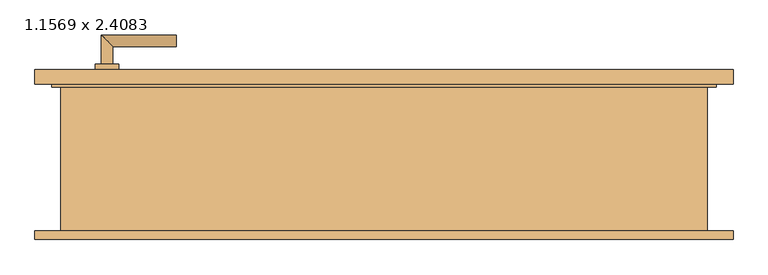
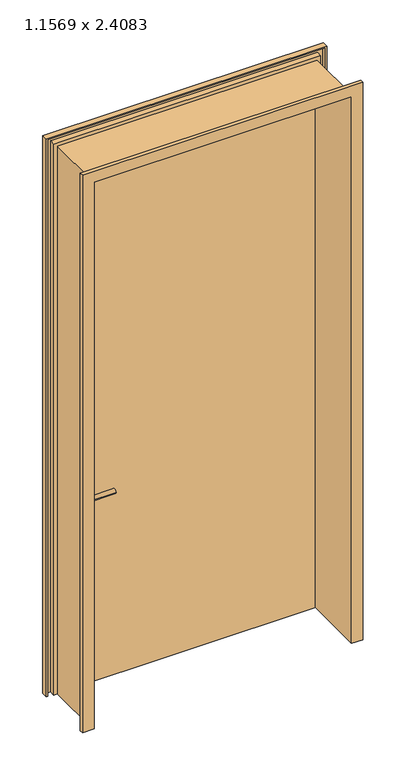
"""IFC4 building model written with IfcOpenShell, lengths in millimetres: door geometry, Drehflügel 1-flg - Stahlzarge : 1.1569 x 2.4083."""

from ifc_helpers import new_model, si_unit, point, frame, frame_2d, origin, place, context, project, spatial, polyline, circle_curve, ellipse_curve, trimmed, segment, composite_curve, outline, extrude, faceted_brep, source, transform, mapped, element, save
from ifc_brep_helpers import plane_surface, cylinder_surface, advanced_brep


def door_1_1569_x_2_4083_937cce7c(model_context):
    return source(origin(), model_context, "Body", "SolidModel", [
        advanced_brep(
        [(-488.45, 116.4346141, 1000.0), (-468.45, 116.4346141, 1000.0), (-488.45, 46.4346141, 1000.0), (-468.45, 66.4346141, 1000.0), (-358.45, 46.4346141, 1000.0), (-358.45, 66.4346141, 1000.0)],
        [
            (0, 1, circle_curve(frame((-478.45, 116.4346141, 1000.0), z_axis=(0.0, 1.0, 0.0), x_axis=(1.0, 0.0, 0.0)), 10.0)),
            (1, 0, circle_curve(frame((-478.45, 116.4346141, 1000.0), z_axis=(0.0, 1.0, 0.0), x_axis=(1.0, 0.0, 0.0)), 10.0)),
            (0, 2),
            (2, 3, ellipse_curve(frame((-478.45, 56.4346141, 1000.0), z_axis=(-0.7071067811865385, 0.7071067811865565, 0.0), x_axis=(0.7071067811865563, 0.7071067811865386, 0.0)), 14.1421356, 10.0)),
            (3, 1),
            (3, 2, ellipse_curve(frame((-478.45, 56.4346141, 1000.0), z_axis=(-0.7071067811865385, 0.7071067811865565, 0.0), x_axis=(0.7071067811865563, 0.7071067811865386, 0.0)), 14.1421356, 10.0)),
            (4, 5, circle_curve(frame((-358.45, 56.4346141, 1000.0), z_axis=(1.0, 0.0, 0.0), x_axis=(0.0, 1.0, 0.0)), 10.0)),
            (5, 4, circle_curve(frame((-358.45, 56.4346141, 1000.0), z_axis=(1.0, 0.0, 0.0), x_axis=(0.0, 1.0, 0.0)), 10.0)),
            (2, 4),
            (5, 3),
        ],
        [
            plane_surface(frame((-478.45, 116.4346141, -287.7526403), z_axis=(0.0, 1.0, 0.0), x_axis=(0.0, 0.0, 1.0))),
            cylinder_surface(frame((-478.45, 116.4346141, 1000.0), z_axis=(0.0, 1.0, 0.0), x_axis=(1.0, 0.0, 0.0)), 10.0),
            plane_surface(frame((-358.45, 56.4346141, -287.7526403), z_axis=(1.0, 0.0, 0.0), x_axis=(0.0, 0.0, 1.0))),
            cylinder_surface(frame((-478.45, 56.4346141, 1000.0), z_axis=(-1.0, 0.0, 0.0), x_axis=(0.0, 1.0, 0.0)), 10.0),
        ],
        [
            (0, [[1, 2]]),
            (1, [[-1, 3, 4, 5]]),
            (1, [[-2, -5, 6, -3]]),
            (2, [[7, 8]]),
            (3, [[-4, 9, -8, 10]]),
            (3, [[-6, -10, -7, -9]]),
        ],
    ),
        advanced_brep(
        [(-468.45, 176.4346141, 1000.0), (-488.45, 176.4346141, 1000.0), (-468.45, 206.4346141, 1000.0), (-488.45, 226.4346141, 1000.0), (-358.45, 206.4346141, 1000.0), (-358.45, 226.4346141, 1000.0)],
        [
            (0, 1, circle_curve(frame((-478.45, 176.4346141, 1000.0), z_axis=(0.0, -1.0, 0.0), x_axis=(-1.0, 0.0, 0.0)), 10.0)),
            (1, 0, circle_curve(frame((-478.45, 176.4346141, 1000.0), z_axis=(0.0, -1.0, 0.0), x_axis=(-1.0, 0.0, 0.0)), 10.0)),
            (0, 2),
            (2, 3, ellipse_curve(frame((-478.45, 216.4346141, 1000.0), z_axis=(-0.7071067811865475, -0.7071067811865475, 0.0), x_axis=(0.7071067811865474, -0.7071067811865476, 0.0)), 14.1421356, 10.0)),
            (3, 1),
            (3, 2, ellipse_curve(frame((-478.45, 216.4346141, 1000.0), z_axis=(-0.7071067811865475, -0.7071067811865475, 0.0), x_axis=(0.7071067811865474, -0.7071067811865476, 0.0)), 14.1421356, 10.0)),
            (4, 5, circle_curve(frame((-358.45, 216.4346141, 1000.0), z_axis=(1.0, 0.0, 0.0), x_axis=(0.0, 1.0, 0.0)), 10.0)),
            (5, 4, circle_curve(frame((-358.45, 216.4346141, 1000.0), z_axis=(1.0, 0.0, 0.0), x_axis=(0.0, 1.0, 0.0)), 10.0)),
            (2, 4),
            (5, 3),
        ],
        [
            plane_surface(frame((-478.45, 176.4346141, -287.7526403), z_axis=(0.0, -1.0, 0.0), x_axis=(0.0, 0.0, 1.0))),
            cylinder_surface(frame((-478.45, 176.4346141, 1000.0), z_axis=(0.0, -1.0, 0.0), x_axis=(-1.0, 0.0, 0.0)), 10.0),
            plane_surface(frame((-358.45, 216.4346141, -287.7526403), z_axis=(1.0, 0.0, 0.0), x_axis=(0.0, 0.0, 1.0))),
            cylinder_surface(frame((-478.45, 216.4346141, 1000.0), z_axis=(-1.0, 0.0, 0.0), x_axis=(0.0, 1.0, 0.0)), 10.0),
        ],
        [
            (0, [[1, 2]]),
            (1, [[-1, 3, 4, 5]]),
            (1, [[-2, -5, 6, -3]]),
            (2, [[7, 8]]),
            (3, [[-4, 9, -8, 10]]),
            (3, [[-6, -10, -7, -9]]),
        ],
    ),
        extrude(outline(composite_curve([segment(trimmed(circle_curve(frame_2d((1000.0, -478.45)), 20.0), [point((1000.0, -498.45))], [point((1000.0, -458.45))], False, "CARTESIAN"), True, "CONTINUOUS"), segment(trimmed(circle_curve(frame_2d((1000.0, -478.45)), 20.0), [point((1000.0, -458.45))], [point((1000.0, -498.45))], False, "CARTESIAN"), True, "CONTINUOUS")], self_intersect=False)), frame((0.0, 106.4346141, 0.0), z_axis=(0.0, 1.0, 0.0), x_axis=(0.0, 0.0, 1.0)), (0.0, 0.0, 1.0), 10.0),
        extrude(outline(composite_curve([segment(trimmed(circle_curve(frame_2d((1000.0, -478.45)), 20.0), [point((1000.0, -498.45))], [point((1000.0, -458.45))], False, "CARTESIAN"), True, "CONTINUOUS"), segment(trimmed(circle_curve(frame_2d((1000.0, -478.45)), 20.0), [point((1000.0, -458.45))], [point((1000.0, -498.45))], False, "CARTESIAN"), True, "CONTINUOUS")], self_intersect=False)), frame((0.0, 166.4346141, 0.0), z_axis=(0.0, 1.0, 0.0), x_axis=(0.0, 0.0, 1.0)), (0.0, 0.0, 1.0), 10.0),
        extrude(outline(polyline([(568.45, 141.4346141), (-568.45, 141.4346141), (-568.45, 166.4346141), (568.45, 166.4346141), (568.45, 141.4346141)])), frame((0.0, 0.0, 100.0), z_axis=(0.0, 0.0, 1.0), x_axis=(1.0, 0.0, 0.0)), (0.0, 0.0, 1.0), 2498.3),
        faceted_brep([(602.9103207, -127.5653859, 100.0), (553.45, -127.5653859, 100.0), (553.45, 141.4346141, 100.0), (568.45, 141.4346141, 100.0), (568.45, 166.4346141, 100.0), (602.9103207, 166.4346141, 100.0), (602.9103207, 141.4346141, 100.0), (597.9103207, 141.4346141, 100.0), (597.9103207, 161.4346141, 100.0), (573.45, 161.4346141, 100.0), (573.45, 136.4346141, 100.0), (558.45, 136.4346141, 100.0), (558.45, -122.5653859, 100.0), (597.9103207, -122.5653859, 100.0), (597.9103207, -112.5653859, 100.0), (602.9103207, -112.5653859, 100.0), (602.9103207, -127.5653859, 2632.7603207), (-602.9103207, -127.5653859, 2632.7603207), (-602.9103207, -127.5653859, 100.0), (-553.45, -127.5653859, 100.0), (-553.45, -127.5653859, 2583.3), (553.45, -127.5653859, 2583.3), (553.45, 141.4346141, 2583.3), (-553.45, 141.4346141, 2583.3), (-553.45, 141.4346141, 100.0), (-568.45, 141.4346141, 100.0), (-568.45, 141.4346141, 2598.3), (568.45, 141.4346141, 2598.3), (568.45, 166.4346141, 2598.3), (-568.45, 166.4346141, 2598.3), (-568.45, 166.4346141, 100.0), (-602.9103207, 166.4346141, 100.0), (-602.9103207, 166.4346141, 2632.7603207), (602.9103207, 166.4346141, 2632.7603207), (602.9103207, 141.4346141, 2632.7603207), (-602.9103207, 141.4346141, 2632.7603207), (-602.9103207, 141.4346141, 100.0), (-597.9103207, 141.4346141, 100.0), (-597.9103207, 141.4346141, 2627.7603207), (597.9103207, 141.4346141, 2627.7603207), (597.9103207, 161.4346141, 2627.7603207), (-597.9103207, 161.4346141, 2627.7603207), (-597.9103207, 161.4346141, 100.0), (-573.45, 161.4346141, 100.0), (-573.45, 161.4346141, 2603.3), (573.45, 161.4346141, 2603.3), (573.45, 136.4346141, 2603.3), (-573.45, 136.4346141, 2603.3), (-573.45, 136.4346141, 100.0), (-558.45, 136.4346141, 100.0), (-558.45, 136.4346141, 2588.3), (558.45, 136.4346141, 2588.3), (558.45, -122.5653859, 2588.3), (-558.45, -122.5653859, 2588.3), (-558.45, -122.5653859, 100.0), (-597.9103207, -122.5653859, 100.0), (-597.9103207, -122.5653859, 2627.7603207), (597.9103207, -122.5653859, 2627.7603207), (597.9103207, -112.5653859, 2627.7603207), (-597.9103207, -112.5653859, 2627.7603207), (-597.9103207, -112.5653859, 100.0), (-602.9103207, -112.5653859, 100.0), (-602.9103207, -112.5653859, 2632.7603207), (602.9103207, -112.5653859, 2632.7603207)], [[[0, 1, 2, 3, 4, 5, 6, 7, 8, 9, 10, 11, 12, 13, 14, 15]], [[1, 0, 16, 17, 18, 19, 20, 21]], [[2, 1, 21, 22]], [[3, 2, 22, 23, 24, 25, 26, 27]], [[4, 3, 27, 28]], [[5, 4, 28, 29, 30, 31, 32, 33]], [[6, 5, 33, 34]], [[7, 6, 34, 35, 36, 37, 38, 39]], [[8, 7, 39, 40]], [[9, 8, 40, 41, 42, 43, 44, 45]], [[10, 9, 45, 46]], [[11, 10, 46, 47, 48, 49, 50, 51]], [[12, 11, 51, 52]], [[13, 12, 52, 53, 54, 55, 56, 57]], [[14, 13, 57, 58]], [[15, 14, 58, 59, 60, 61, 62, 63]], [[0, 15, 63, 16]], [[17, 62, 61, 18]], [[18, 61, 60, 55, 54, 49, 48, 43, 42, 37, 36, 31, 30, 25, 24, 19]], [[23, 20, 19, 24]], [[29, 26, 25, 30]], [[35, 32, 31, 36]], [[41, 38, 37, 42]], [[47, 44, 43, 48]], [[53, 50, 49, 54]], [[59, 56, 55, 60]], [[22, 21, 20, 23]], [[28, 27, 26, 29]], [[34, 33, 32, 35]], [[40, 39, 38, 41]], [[46, 45, 44, 47]], [[52, 51, 50, 53]], [[58, 57, 56, 59]], [[16, 63, 62, 17]]]),
    ])


if __name__ == "__main__":
    model = new_model("IFC4")
    model_context = context("Model", 3, world=origin())
    ifc_project = project(units=[si_unit("LENGTHUNIT", "METRE", prefix="MILLI")], contexts=[model_context])
    site = spatial("IfcSite", under=ifc_project)
    building = spatial("IfcBuilding", under=site)
    placement = place(None, origin())
    door_1_1569_x_2_4083_shape = door_1_1569_x_2_4083_937cce7c(model_context)
    element("IfcDoor", 1, ObjectType="Drehflügel 1-flg - Stahlzarge : 1.1569 x 2.4083", at=placement, inside=building, context=model_context, shape_type="MappedRepresentation", body=[
        mapped(door_1_1569_x_2_4083_shape, transform((0.0, 0.0, 0.0), x_axis=(1.0, 0.0, 0.0), y_axis=(0.0, 1.0, 0.0), z_axis=(0.0, 0.0, 1.0))),
    ])
    save(model, "model.ifc")

# Revit data of these elements
# Type "Drehflügel 1-flg - Stahlzarge : 1.1569 x 2.4083"
#   Type Mark = "22"
#   Operation = "SingleSwingRight"
#   Keynote = "16.03"
#   Analytic Construction = "Metall"
#   Thermal Resistance (R) = 0.270117 (m²·K)/W
#   Heat Transfer Coefficient (U) = 3.7021 W/(m²·K)
#   Rough Width = 1.1569 m
#   Rough Height [instance default] = 2.6083 m
#   Höhe Türgriff [instance default] = 0.900 m
#   Height = 2.5083 m
#   Fußbodenaufbau [instance default] = 0.100 m
#   Width = 1.1569 m
#   Sichtbarkeit Sturzlinien [instance default] = yes
#   Türgriff auswählen [instance default] = element 221079
#   Türgriff [instance default] = none
#   Türflügel [instance default] = none
#   Rahmen/Pfosten [instance default] = Metall - Lackiert - Grau
#   Visual Light Transmittance = 0
#   Solar Heat Gain Coefficient = 0
#   Function = (empty or 0)
#   Wall Closure = (empty or 0)
# Element 1 (IfcDoor, "Drehflügel 1-flg - Stahlzarge : 1.1569 x 2.4083")
#   Materials on its faces: "Metall - Lackiert - Grau", "Metall - Chrom", "Holz - Birke"
# Materials
#   "Metall - Lackiert - Grau": class "Farbe 1", colour RGB 98 98 98, transparency 0, Cost = 0
#   "Metall - Chrom": class "Metall", colour RGB 247 247 247, transparency 0, Cost = 0
#   "Holz - Birke": class "Holz", colour RGB 213 164 103, transparency 0, Cost = 0
